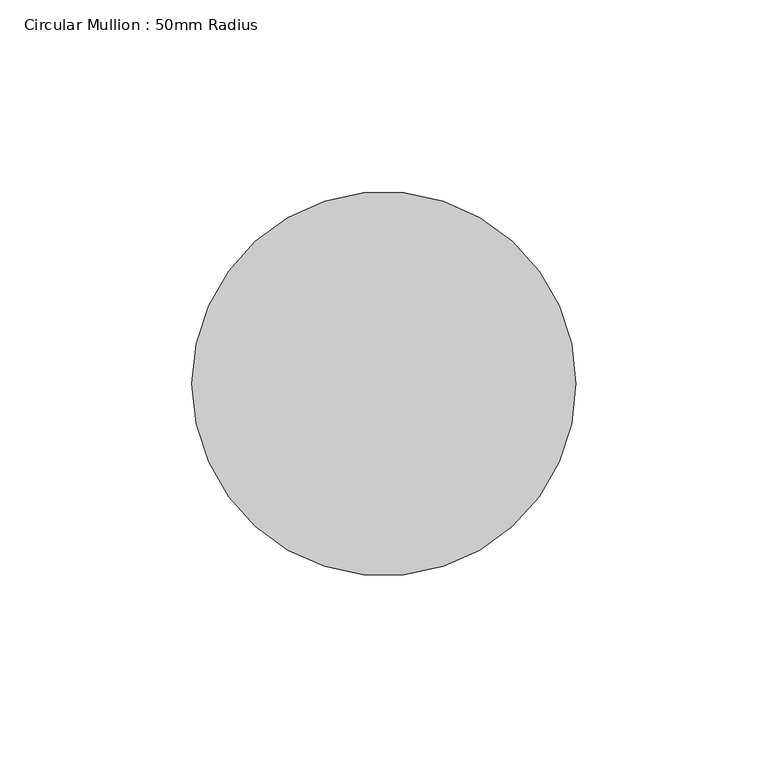
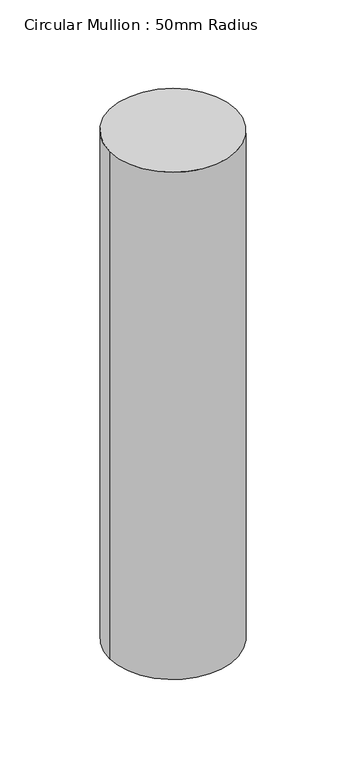
"""IFC4 building model written with IfcOpenShell, lengths in millimetres: member geometry, Circular Mullion : 50mm Radius."""

from ifc_helpers import new_model, si_unit, point, frame, origin, origin_2d, place, context, project, spatial, circle_curve, trimmed, segment, composite_curve, outline, extrude, source, transform, mapped, element, save


def circular_mullion_50mm_radius_afa1f0d7(model_context):
    return source(origin(), model_context, "Body", "SweptSolid", [
        extrude(outline(composite_curve([segment(trimmed(circle_curve(origin_2d(), 50.0), [point((50.0, 0.0))], [point((-50.0, 0.0))], False, "CARTESIAN"), True, "CONTINUOUS"), segment(trimmed(circle_curve(origin_2d(), 50.0), [point((-50.0, 0.0))], [point((50.0, 0.0))], False, "CARTESIAN"), True, "CONTINUOUS")], self_intersect=False)), frame((0.0, 0.0, -423.1698779), z_axis=(0.0, 0.0, 1.0), x_axis=(1.0, 0.0, 0.0)), (0.0, 0.0, 1.0), 423.1698779),
    ])


if __name__ == "__main__":
    model = new_model("IFC4")
    model_context = context("Model", 3, world=origin())
    ifc_project = project(units=[si_unit("LENGTHUNIT", "METRE", prefix="MILLI")], contexts=[model_context])
    site = spatial("IfcSite", under=ifc_project)
    building = spatial("IfcBuilding", under=site)
    placement = place(None, origin())
    circular_mullion_50mm_radius_shape = circular_mullion_50mm_radius_afa1f0d7(model_context)
    element("IfcMember", 1, ObjectType="Circular Mullion : 50mm Radius", at=placement, inside=building, context=model_context, shape_type="MappedRepresentation", body=[
        mapped(circular_mullion_50mm_radius_shape, transform((0.0, 0.0, 0.0), x_axis=(1.0, 0.0, 0.0), y_axis=(0.0, 1.0, 0.0), z_axis=(0.0, 0.0, 1.0))),
    ])
    save(model, "model.ifc")

# Revit data of these elements
# Type "Circular Mullion : 50mm Radius"
#   built-in parameter 1007350 = 0.164042 (stored number, unit not read)
# Element 1 (IfcMember, "Circular Mullion : 50mm Radius")
#   Materials on its faces: "Aluminium"
# Materials
#   "Aluminium": class "Metal", colour RGB 247 247 247, transparency 0, Description = "Aluminium 6061", Cost = 0
